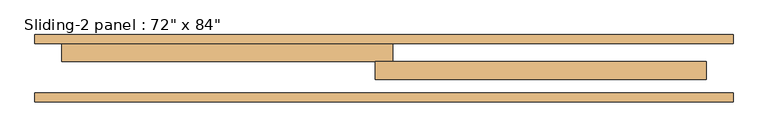
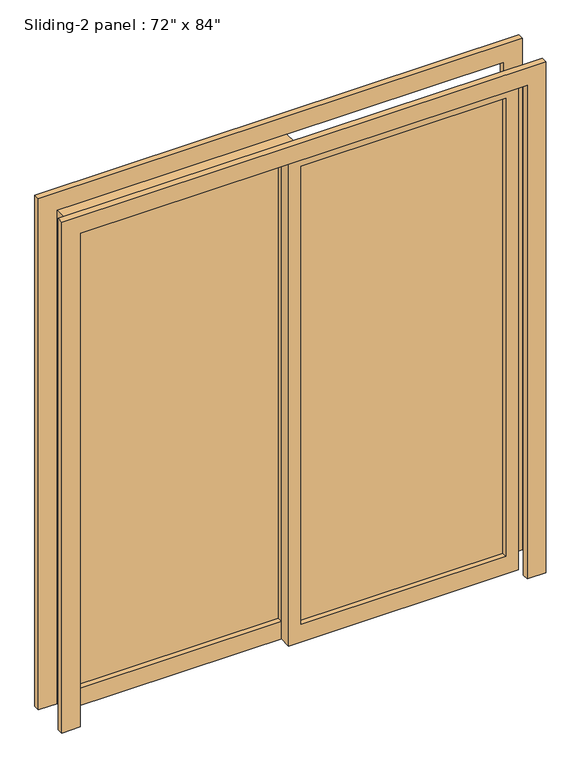
"""IFC4 building model written with IfcOpenShell, lengths in millimetres: door geometry."""

from ifc_helpers import new_model, si_unit, frame, origin, place, context, project, spatial, polyline, outline, extrude, source, transform, mapped, element, save


def door_a33c1234(model_context):
    return source(origin(), model_context, "Body", "SweptSolid", [
        extrude(outline(polyline([(25.4, 123.825), (863.6, 123.825), (863.6, 117.475), (25.4, 117.475), (25.4, 123.825)])), frame((0.0, 0.0, 76.2), z_axis=(0.0, 0.0, 1.0), x_axis=(1.0, 0.0, 0.0)), (0.0, 0.0, 1.0), 1981.2),
        extrude(outline(polyline([(2133.6, -25.4), (0.0, -25.4), (0.0, 914.4), (2133.6, 914.4), (2133.6, -25.4)]), holes=[polyline([(2057.4, 25.4), (2057.4, 863.6), (76.2, 863.6), (76.2, 25.4), (2057.4, 25.4)])]), frame((0.0, 95.25, 0.0), z_axis=(0.0, 1.0, 0.0), x_axis=(0.0, 0.0, 1.0)), (0.0, 0.0, 1.0), 50.8),
        extrude(outline(polyline([(-863.6, 174.625), (-25.4, 174.625), (-25.4, 168.275), (-863.6, 168.275), (-863.6, 174.625)])), frame((0.0, 0.0, 76.2), z_axis=(0.0, 0.0, 1.0), x_axis=(1.0, 0.0, 0.0)), (0.0, 0.0, 1.0), 1981.2),
        extrude(outline(polyline([(2133.6, 25.4), (2133.6, -914.4), (0.0, -914.4), (0.0, 25.4), (2133.6, 25.4)]), holes=[polyline([(2057.4, -25.4), (76.2, -25.4), (76.2, -863.6), (2057.4, -863.6), (2057.4, -25.4)])]), frame((0.0, 146.05, 0.0), z_axis=(0.0, 1.0, 0.0), x_axis=(0.0, 0.0, 1.0)), (0.0, 0.0, 1.0), 50.8),
        extrude(outline(polyline([(0.0, -990.6), (0.0, -914.4), (2133.6, -914.4), (2133.6, 914.4), (0.0, 914.4), (0.0, 990.6), (2209.8, 990.6), (2209.8, -990.6), (0.0, -990.6)])), frame((0.0, 31.75, 0.0), z_axis=(0.0, 1.0, 0.0), x_axis=(0.0, 0.0, 1.0)), (0.0, 0.0, 1.0), 25.4),
        extrude(outline(polyline([(0.0, 990.6), (2209.8, 990.6), (2209.8, -990.6), (0.0, -990.6), (0.0, -914.4), (2133.6, -914.4), (2133.6, 914.4), (0.0, 914.4), (0.0, 990.6)])), frame((0.0, 196.85, 0.0), z_axis=(0.0, 1.0, 0.0), x_axis=(0.0, 0.0, 1.0)), (0.0, 0.0, 1.0), 25.4),
    ])


if __name__ == "__main__":
    model = new_model("IFC4")
    model_context = context("Model", 3, world=origin())
    ifc_project = project(units=[si_unit("LENGTHUNIT", "METRE", prefix="MILLI")], contexts=[model_context])
    site = spatial("IfcSite", under=ifc_project)
    building = spatial("IfcBuilding", under=site)
    placement = place(None, origin())
    door_shape = door_a33c1234(model_context)
    element("IfcDoor", 1, ObjectType="Sliding-2 panel : 72\" x 84\"", at=placement, inside=building, context=model_context, shape_type="MappedRepresentation", body=[
        mapped(door_shape, transform((0.0, 0.0, 0.0), x_axis=(1.0, 0.0, 0.0), y_axis=(0.0, 1.0, 0.0), z_axis=(0.0, 0.0, 1.0))),
    ])
    save(model, "model.ifc")

# Revit data of these elements
# Type "Sliding-2 panel : 72\" x 84\""
#   Type Mark = "1"
#   Assembly Code = "C1020"
#   Thickness = 0' - 2"
#   Height = 7' - 0"
#   Rail Width = 0' - 3"
#   Stile Width = 0' - 2"
#   Trim Projection Ext = 0' - 1"
#   Trim Projection Int = 0' - 1"
#   Trim Width = 0' - 3"
#   Width = 6' - 0"
#   Function = 0
#   Door Material = Door - Panel
#   Frame Material = Door - Frame
#   Wall Closure = (empty or 0)
# Element 1 (IfcDoor, "Sliding-2 panel : 72\" x 84\"")
#   Materials on its faces: "Door - Panel", "Door - Frame", "Glass"
# Materials
#   "Door - Panel": class "Wood", colour RGB 149 143 132, transparency 0, Comments = "Rendering appearance not upgraded Rendering appearance not upgraded "
#   "Door - Frame": class "Unassigned", colour RGB 118 70 51, transparency 0, Comments = "Rendering appearance not upgraded Rendering appearance not upgraded "
#   "Glass": class "Glass", colour RGB 218 227 224, transparency 0.7, Comments = "Rendering appearance not upgraded Rendering appearance not upgraded ", Description = "Glass"
